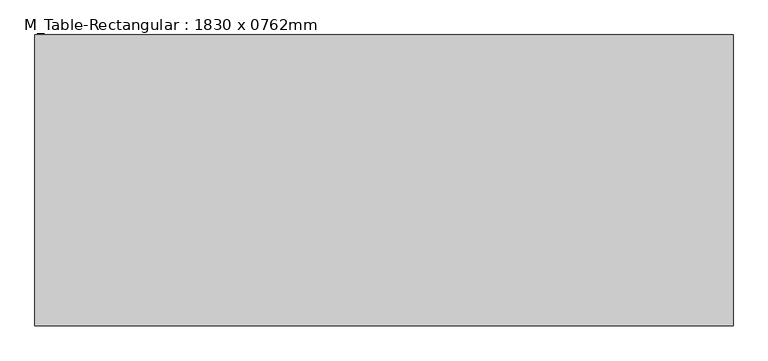
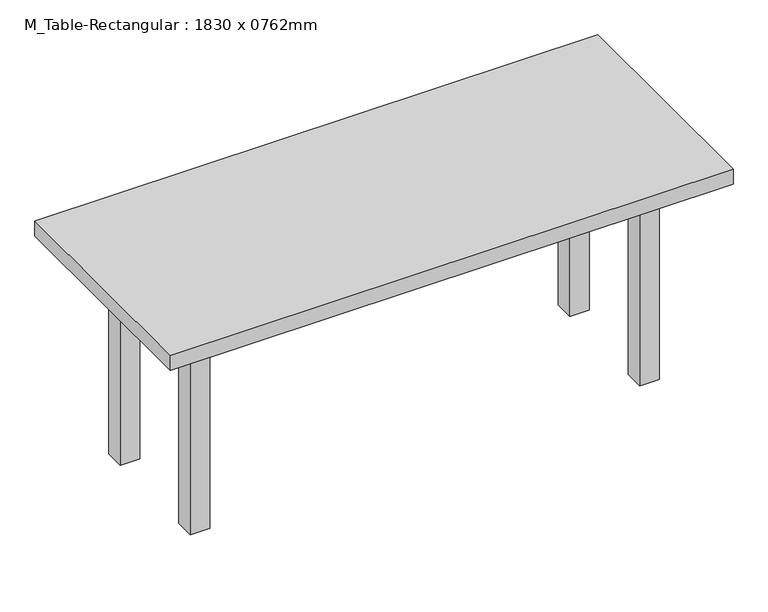
"""IFC4 building model written with IfcOpenShell, lengths in millimetres: furniture geometry, M_Table-Rectangular : 1830 x 0762mm."""

from ifc_helpers import new_model, si_unit, frame, origin, origin_with_axes, place, context, project, spatial, polyline, outline, extrude, source, transform, mapped, element, save


def m_table_rectangular_1830_x_0762mm_ec068ed4(model_context):
    return source(origin(), model_context, "Body", "SweptSolid", [
        extrude(outline(polyline([(699.1, -190.5), (-699.1, -190.5), (-699.1, -165.1), (699.1, -165.1), (699.1, -190.5)])), frame((0.0, 0.0, 609.6), z_axis=(0.0, 0.0, 1.0), x_axis=(1.0, 0.0, 0.0)), (0.0, 0.0, 1.0), 101.6),
        extrude(outline(polyline([(699.1, 190.5), (699.1, 165.1), (-699.1, 165.1), (-699.1, 190.5), (699.1, 190.5)])), frame((0.0, 0.0, 609.6), z_axis=(0.0, 0.0, 1.0), x_axis=(1.0, 0.0, 0.0)), (0.0, 0.0, 1.0), 101.6),
        extrude(outline(polyline([(-711.8, 165.1), (-711.8, -165.1), (-737.2, -165.1), (-737.2, 165.1), (-711.8, 165.1)])), frame((0.0, 0.0, 609.6), z_axis=(0.0, 0.0, 1.0), x_axis=(1.0, 0.0, 0.0)), (0.0, 0.0, 1.0), 101.6),
        extrude(outline(polyline([(711.8, 165.1), (737.2, 165.1), (737.2, -165.1), (711.8, -165.1), (711.8, 165.1)])), frame((0.0, 0.0, 609.6), z_axis=(0.0, 0.0, 1.0), x_axis=(1.0, 0.0, 0.0)), (0.0, 0.0, 1.0), 101.6),
        extrude(outline(polyline([(915.0, -381.0), (-915.0, -381.0), (-915.0, 381.0), (915.0, 381.0), (915.0, -381.0)])), frame((0.0, 0.0, 711.2), z_axis=(0.0, 0.0, 1.0), x_axis=(1.0, 0.0, 0.0)), (0.0, 0.0, 1.0), 50.8),
        extrude(outline(polyline([(-699.1, -228.6), (-762.6, -228.6), (-762.6, -165.1), (-699.1, -165.1), (-699.1, -228.6)])), origin_with_axes(), (0.0, 0.0, 1.0), 711.2),
        extrude(outline(polyline([(699.1, -228.6), (699.1, -165.1), (762.6, -165.1), (762.6, -228.6), (699.1, -228.6)])), origin_with_axes(), (0.0, 0.0, 1.0), 711.2),
        extrude(outline(polyline([(-699.1, 228.6), (-699.1, 165.1), (-762.6, 165.1), (-762.6, 228.6), (-699.1, 228.6)])), origin_with_axes(), (0.0, 0.0, 1.0), 711.2),
        extrude(outline(polyline([(699.1, 228.6), (762.6, 228.6), (762.6, 165.1), (699.1, 165.1), (699.1, 228.6)])), origin_with_axes(), (0.0, 0.0, 1.0), 711.2),
    ])


if __name__ == "__main__":
    model = new_model("IFC4")
    model_context = context("Model", 3, world=origin())
    ifc_project = project(units=[si_unit("LENGTHUNIT", "METRE", prefix="MILLI")], contexts=[model_context])
    site = spatial("IfcSite", under=ifc_project)
    building = spatial("IfcBuilding", under=site)
    placement = place(None, origin())
    m_table_rectangular_1830_x_0762mm_shape = m_table_rectangular_1830_x_0762mm_ec068ed4(model_context)
    element("IfcFurniture", 1, ObjectType="M_Table-Rectangular : 1830 x 0762mm", at=placement, inside=building, context=model_context, shape_type="MappedRepresentation", body=[
        mapped(m_table_rectangular_1830_x_0762mm_shape, transform((0.0, 0.0, 0.0), x_axis=(1.0, 0.0, 0.0), y_axis=(0.0, 1.0, 0.0), z_axis=(0.0, 0.0, 1.0))),
    ])
    save(model, "model.ifc")

# Revit data of these elements
# Type "M_Table-Rectangular : 1830 x 0762mm"
#   Height = 762 mm
#   Length = 1830 mm
#   Width = 762 mm
#   Base Material = Birch
#   Top Material = Birch
#   Default Elevation = 0
# Element 1 (IfcFurniture, "M_Table-Rectangular : 1830 x 0762mm")
#   Materials on its faces: "Birch"
# Materials
#   "Birch": class "Wood", colour RGB 224 178 126, transparency 0, Description = "Betula Alleghaniensis", Cost = 0
